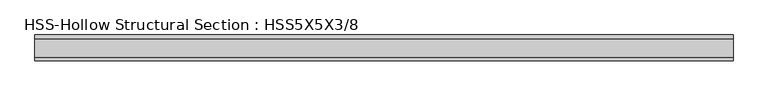
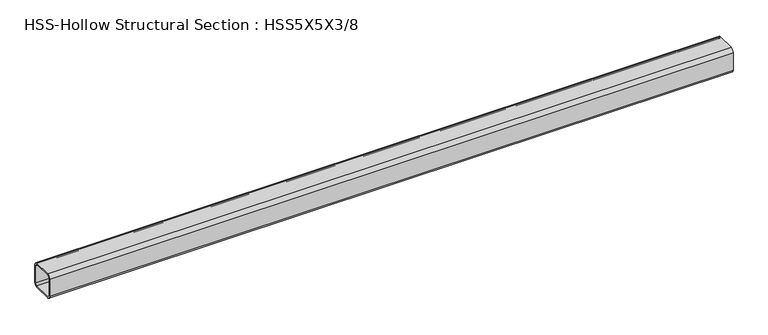
"""IFC4 building model written with IfcOpenShell, lengths in millimetres: member geometry, HSS-Hollow Structural Section : HSS5X5X3/8."""

from ifc_helpers import new_model, si_unit, point, frame, frame_2d, origin, place, context, project, spatial, polyline, circle_curve, trimmed, segment, composite_curve, outline, extrude, source, transform, mapped, element, save


def hss_hollow_structural_section_hss5x5x3_8_c527732f(model_context):
    return source(origin(), model_context, "Body", "SweptSolid", [
        extrude(outline(composite_curve([segment(polyline([(63.5, 45.7708), (63.5, -45.7708)]), True, "CONTINUOUS"), segment(trimmed(circle_curve(frame_2d((45.7708, -45.7708)), 17.7292), [point((63.5, -45.7708))], [point((45.7708, -63.5))], False, "CARTESIAN"), True, "CONTINUOUS"), segment(polyline([(45.7708, -63.5), (-45.7708, -63.5)]), True, "CONTINUOUS"), segment(trimmed(circle_curve(frame_2d((-45.7708, -45.7708)), 17.7292), [point((-45.7708, -63.5))], [point((-63.5, -45.7708))], False, "CARTESIAN"), True, "CONTINUOUS"), segment(polyline([(-63.5, -45.7708), (-63.5, 45.7708)]), True, "CONTINUOUS"), segment(trimmed(circle_curve(frame_2d((-45.7708, 45.7708)), 17.7292), [point((-63.5, 45.7708))], [point((-45.7708, 63.5))], False, "CARTESIAN"), True, "CONTINUOUS"), segment(polyline([(-45.7708, 63.5), (45.7708, 63.5)]), True, "CONTINUOUS"), segment(trimmed(circle_curve(frame_2d((45.7708, 45.7708)), 17.7292), [point((45.7708, 63.5))], [point((63.5, 45.7708))], False, "CARTESIAN"), True, "CONTINUOUS")], self_intersect=False), holes=[composite_curve([segment(trimmed(circle_curve(frame_2d((-45.7708, 45.7708)), 8.8646), [point((-45.7708, 54.6354))], [point((-54.6354, 45.7708))], True, "CARTESIAN"), True, "CONTINUOUS"), segment(polyline([(-54.6354, 45.7708), (-54.6354, -45.7708)]), True, "CONTINUOUS"), segment(trimmed(circle_curve(frame_2d((-45.7708, -45.7708)), 8.8646), [point((-54.6354, -45.7708))], [point((-45.7708, -54.6354))], True, "CARTESIAN"), True, "CONTINUOUS"), segment(polyline([(-45.7708, -54.6354), (45.7708, -54.6354)]), True, "CONTINUOUS"), segment(trimmed(circle_curve(frame_2d((45.7708, -45.7708)), 8.8646), [point((45.7708, -54.6354))], [point((54.6354, -45.7708))], True, "CARTESIAN"), True, "CONTINUOUS"), segment(polyline([(54.6354, -45.7708), (54.6354, 45.7708)]), True, "CONTINUOUS"), segment(trimmed(circle_curve(frame_2d((45.7708, 45.7708)), 8.8646), [point((54.6354, 45.7708))], [point((45.7708, 54.6354))], True, "CARTESIAN"), True, "CONTINUOUS"), segment(polyline([(45.7708, 54.6354), (-45.7708, 54.6354)]), True, "CONTINUOUS")], self_intersect=False)]), frame((-1676.7459948, 0.0, 0.0), z_axis=(1.0, 0.0, 0.0), x_axis=(0.0, 1.0, 0.0)), (0.0, 0.0, 1.0), 3423.5379874),
    ])


if __name__ == "__main__":
    model = new_model("IFC4")
    model_context = context("Model", 3, world=origin())
    ifc_project = project(units=[si_unit("LENGTHUNIT", "METRE", prefix="MILLI")], contexts=[model_context])
    site = spatial("IfcSite", under=ifc_project)
    building = spatial("IfcBuilding", under=site)
    placement = place(None, origin())
    hss_hollow_structural_section_hss5x5x3_8_shape = hss_hollow_structural_section_hss5x5x3_8_c527732f(model_context)
    element("IfcMember", 1, ObjectType="HSS-Hollow Structural Section : HSS5X5X3/8", at=placement, inside=building, context=model_context, shape_type="MappedRepresentation", body=[
        mapped(hss_hollow_structural_section_hss5x5x3_8_shape, transform((0.0, 0.0, 0.0), x_axis=(1.0, 0.0, 0.0), y_axis=(0.0, 1.0, 0.0), z_axis=(0.0, 0.0, 1.0))),
    ])
    save(model, "model.ifc")

# Revit data of these elements
# Type "HSS-Hollow Structural Section : HSS5X5X3/8"
#   Assembly Code = "B10"
#   Shape = "Square"
#   W = 22.3
#   Ht = 0' - 5"
#   Length [instance default] = 5' - 0"
#   b = 0' - 5"
#   kr = 0' - 0.698"
#   t = 0' - 0.349"
#   A = 0.0429167 SF
#   Structural Material [instance default] = Steel ASTM A500, Grade B, Rectangular and Square
# Element 1 (IfcMember, "HSS-Hollow Structural Section : HSS5X5X3/8")
#   Materials on its faces: "Steel ASTM A500, Grade B, Rectangular and Square"
# Materials
#   "Steel ASTM A500, Grade B, Rectangular and Square": class "Metal", colour RGB 199 199 199, transparency 0, Description = "Carbon steel", Cost = 0
